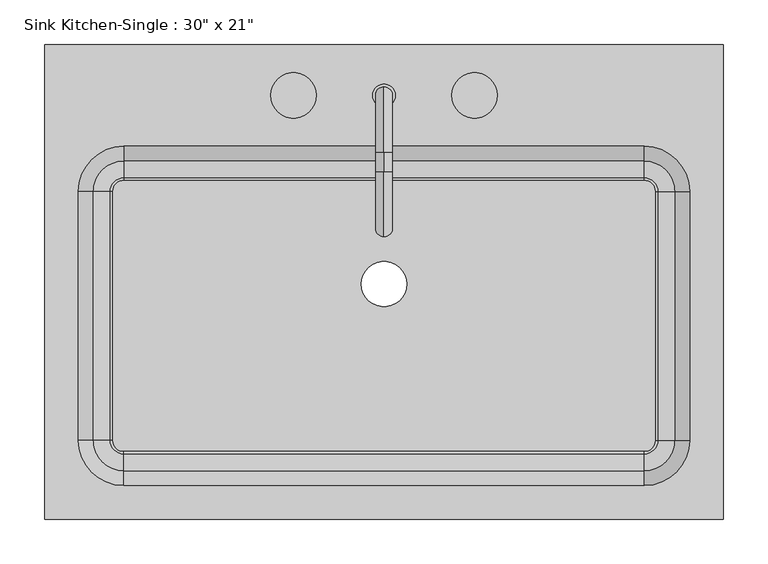
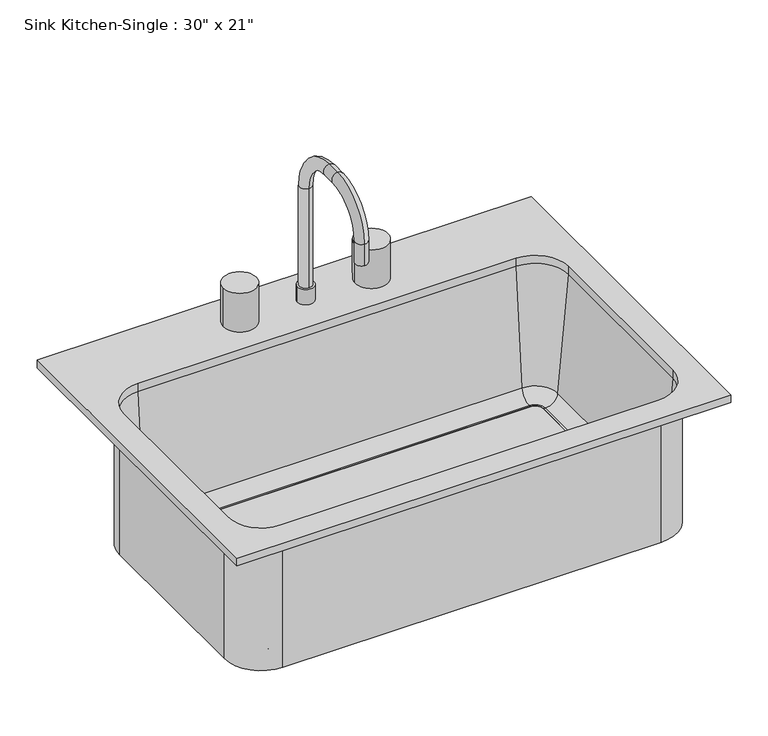
"""IFC4 building model written with IfcOpenShell, lengths in millimetres: flow terminal geometry."""

from ifc_helpers import new_model, si_unit, point, frame, frame_2d, origin, place, context, project, spatial, polyline, circle_curve, ellipse_curve, trimmed, segment, composite_curve, outline, extrude, source, transform, mapped, element, save
from ifc_brep_helpers import plane_surface, cylinder_surface, revolved_surface, advanced_brep


def flow_terminal_38af2918(model_context):
    return source(origin(), model_context, "Body", "SolidModel", [
        advanced_brep(
        [(396.6892406, 269.0454011, 927.1), (-365.3107594, 269.0454011, 927.1), (-365.3107594, -264.3545989, 927.1), (396.6892406, -264.3545989, 927.1), (307.7892406, 154.7454011, 927.1), (358.5892406, 103.9454011, 927.1), (358.5892406, -175.4545989, 927.1), (307.7892406, -226.2545989, 927.1), (-276.4107594, -226.2545989, 927.1), (-327.2107594, -175.4545989, 927.1), (-327.2107594, 103.9454011, 927.1), (-276.4107594, 154.7454011, 927.1), (396.6892406, 269.0454011, 914.4), (396.6892406, -264.3545989, 914.4), (-365.3107594, -264.3545989, 914.4), (-365.3107594, 269.0454011, 914.4), (364.9392406, 103.9454011, 914.4), (307.7892406, 161.0954011, 914.4), (-276.4107594, 161.0954011, 914.4), (-333.5607594, 103.9454011, 914.4), (-333.5607594, -175.4545989, 914.4), (-276.4107594, -232.6045989, 914.4), (307.7892406, -232.6045989, 914.4), (364.9392406, -175.4545989, 914.4), (307.7892406, 154.7454011, 914.4), (358.5892406, 103.9454011, 914.4), (358.5892406, -175.4545989, 914.4), (307.7892406, -226.2545989, 914.4), (-276.4107594, -226.2545989, 914.4), (-327.2107594, -175.4545989, 914.4), (-327.2107594, 103.9454011, 914.4), (-276.4107594, 154.7454011, 914.4), (364.9392406, 103.9454011, 698.5), (307.7892406, 161.0954011, 698.5), (320.4892406, 103.9454011, 698.5), (307.7892406, 116.6454011, 698.5), (320.4892406, 103.9454011, 708.025), (307.7892406, 116.6454011, 708.025), (323.0776588, 103.9454011, 708.025), (307.7892406, 119.2338193, 708.025), (342.0551678, 103.9454011, 725.4146831), (307.7892406, 138.2113283, 725.4146831), (364.9392406, -175.4545989, 698.5), (320.4892406, -175.4545989, 698.5), (320.4892406, -175.4545989, 708.025), (323.0776588, -175.4545989, 708.025), (342.0551678, -175.4545989, 725.4146831), (307.7892406, -232.6045989, 698.5), (307.7892406, -188.1545989, 698.5), (307.7892406, -188.1545989, 708.025), (307.7892406, -190.7430171, 708.025), (307.7892406, -209.7205261, 725.4146831), (-276.4107594, -232.6045989, 698.5), (-276.4107594, -188.1545989, 698.5), (-276.4107594, -188.1545989, 708.025), (-276.4107594, -190.7430171, 708.025), (-276.4107594, -209.7205261, 725.4146831), (-333.5607594, -175.4545989, 698.5), (-289.1107594, -175.4545989, 698.5), (-289.1107594, -175.4545989, 708.025), (-291.6991776, -175.4545989, 708.025), (-310.6766866, -175.4545989, 725.4146831), (-333.5607594, 103.9454011, 698.5), (-289.1107594, 103.9454011, 698.5), (-289.1107594, 103.9454011, 708.025), (-291.6991776, 103.9454011, 708.025), (-310.6766866, 103.9454011, 725.4146831), (-276.4107594, 161.0954011, 698.5), (-276.4107594, 116.6454011, 698.5), (-276.4107594, 116.6454011, 708.025), (-276.4107594, 119.2338193, 708.025), (-276.4107594, 138.2113283, 725.4146831)],
        [
            (0, 1),
            (1, 2),
            (2, 3),
            (3, 0),
            (4, 5, circle_curve(frame((307.7892406, 103.9454011, 927.1), z_axis=(0.0, 0.0, -1.0), x_axis=(1.0, 0.0, 0.0)), 50.8)),
            (5, 6),
            (6, 7, circle_curve(frame((307.7892406, -175.4545989, 927.1), z_axis=(0.0, 0.0, -1.0), x_axis=(1.0, 0.0, 0.0)), 50.8)),
            (7, 8),
            (8, 9, circle_curve(frame((-276.4107594, -175.4545989, 927.1), z_axis=(0.0, 0.0, -1.0), x_axis=(1.0, 0.0, 0.0)), 50.8)),
            (9, 10),
            (10, 11, circle_curve(frame((-276.4107594, 103.9454011, 927.1), z_axis=(0.0, 0.0, -1.0), x_axis=(1.0, 0.0, 0.0)), 50.8)),
            (11, 4),
            (12, 13),
            (13, 14),
            (14, 15),
            (15, 12),
            (16, 17, circle_curve(frame((307.7892406, 103.9454011, 914.4), z_axis=(0.0, 0.0, 1.0), x_axis=(0.0, 1.0, 0.0)), 57.15)),
            (17, 18),
            (18, 19, circle_curve(frame((-276.4107594, 103.9454011, 914.4), z_axis=(0.0, 0.0, 1.0), x_axis=(-1.0, 0.0, 0.0)), 57.15)),
            (19, 20),
            (20, 21, circle_curve(frame((-276.4107594, -175.4545989, 914.4), z_axis=(0.0, 0.0, 1.0), x_axis=(0.0, -1.0, 0.0)), 57.15)),
            (21, 22),
            (22, 23, circle_curve(frame((307.7892406, -175.4545989, 914.4), z_axis=(0.0, 0.0, 1.0), x_axis=(1.0, 0.0, 0.0)), 57.15)),
            (23, 16),
            (0, 12),
            (15, 1),
            (14, 2),
            (13, 3),
            (4, 24),
            (24, 25, circle_curve(frame((307.7892406, 103.9454011, 914.4), z_axis=(0.0, 0.0, -1.0), x_axis=(1.0, 0.0, 0.0)), 50.8)),
            (25, 5),
            (25, 26),
            (26, 6),
            (26, 27, circle_curve(frame((307.7892406, -175.4545989, 914.4), z_axis=(0.0, 0.0, -1.0), x_axis=(1.0, 0.0, 0.0)), 50.8)),
            (27, 7),
            (27, 28),
            (28, 8),
            (28, 29, circle_curve(frame((-276.4107594, -175.4545989, 914.4), z_axis=(0.0, 0.0, -1.0), x_axis=(1.0, 0.0, 0.0)), 50.8)),
            (29, 9),
            (29, 30),
            (30, 10),
            (30, 31, circle_curve(frame((-276.4107594, 103.9454011, 914.4), z_axis=(0.0, 0.0, -1.0), x_axis=(1.0, 0.0, 0.0)), 50.8)),
            (31, 11),
            (31, 24),
            (32, 33, circle_curve(frame((307.7892406, 103.9454011, 698.5), z_axis=(0.0, 0.0, 1.0), x_axis=(0.0, 1.0, 0.0)), 57.15)),
            (33, 17),
            (16, 32),
            (32, 34),
            (34, 35, circle_curve(frame((307.7892406, 103.9454011, 698.5), z_axis=(0.0, 0.0, 1.0), x_axis=(0.0, 1.0, 0.0)), 12.7)),
            (35, 33),
            (34, 36),
            (36, 37, circle_curve(frame((307.7892406, 103.9454011, 708.025), z_axis=(0.0, 0.0, 1.0), x_axis=(0.0, 1.0, 0.0)), 12.7)),
            (37, 35),
            (36, 38),
            (38, 39, circle_curve(frame((307.7892406, 103.9454011, 708.025), z_axis=(0.0, 0.0, 1.0), x_axis=(0.0, 1.0, 0.0)), 15.2884182)),
            (39, 37),
            (38, 40, circle_curve(frame((323.0776588, 103.9454011, 727.075), z_axis=(0.0, -1.0, 0.0), x_axis=(1.0, 0.0, 0.0)), 19.05)),
            (40, 41, circle_curve(frame((307.7892406, 103.9454011, 725.4146831), z_axis=(0.0, 0.0, 1.0), x_axis=(0.0, 1.0, 0.0)), 34.2659272)),
            (41, 39, circle_curve(frame((307.7892406, 119.2338193, 727.075), z_axis=(-1.0, 0.0, 0.0), x_axis=(0.0, 1.0, 0.0)), 19.05)),
            (40, 25),
            (24, 41),
            (23, 42),
            (42, 32),
            (42, 43),
            (43, 34),
            (43, 44),
            (44, 36),
            (44, 45),
            (45, 38),
            (45, 46, circle_curve(frame((323.0776588, -175.4545989, 727.075), z_axis=(0.0, -1.0, 0.0), x_axis=(1.0, 0.0, 0.0)), 19.05)),
            (46, 40),
            (46, 26),
            (22, 47),
            (47, 42, circle_curve(frame((307.7892406, -175.4545989, 698.5), z_axis=(0.0, 0.0, 1.0), x_axis=(1.0, 0.0, 0.0)), 57.15)),
            (47, 48),
            (48, 43, circle_curve(frame((307.7892406, -175.4545989, 698.5), z_axis=(0.0, 0.0, 1.0), x_axis=(1.0, 0.0, 0.0)), 12.7)),
            (48, 49),
            (49, 44, circle_curve(frame((307.7892406, -175.4545989, 708.025), z_axis=(0.0, 0.0, 1.0), x_axis=(1.0, 0.0, 0.0)), 12.7)),
            (49, 50),
            (50, 45, circle_curve(frame((307.7892406, -175.4545989, 708.025), z_axis=(0.0, 0.0, 1.0), x_axis=(1.0, 0.0, 0.0)), 15.2884182)),
            (50, 51, circle_curve(frame((307.7892406, -190.7430171, 727.075), z_axis=(-1.0, 0.0, 0.0), x_axis=(0.0, -1.0, 0.0)), 19.05)),
            (51, 46, circle_curve(frame((307.7892406, -175.4545989, 725.4146831), z_axis=(0.0, 0.0, 1.0), x_axis=(1.0, 0.0, 0.0)), 34.2659272)),
            (51, 27),
            (21, 52),
            (52, 47),
            (52, 53),
            (53, 48),
            (53, 54),
            (54, 49),
            (54, 55),
            (55, 50),
            (55, 56, circle_curve(frame((-276.4107594, -190.7430171, 727.075), z_axis=(-1.0, 0.0, 0.0), x_axis=(0.0, -1.0, 0.0)), 19.05)),
            (56, 51),
            (56, 28),
            (20, 57),
            (57, 52, circle_curve(frame((-276.4107594, -175.4545989, 698.5), z_axis=(0.0, 0.0, 1.0), x_axis=(0.0, -1.0, 0.0)), 57.15)),
            (57, 58),
            (58, 53, circle_curve(frame((-276.4107594, -175.4545989, 698.5), z_axis=(0.0, 0.0, 1.0), x_axis=(0.0, -1.0, 0.0)), 12.7)),
            (58, 59),
            (59, 54, circle_curve(frame((-276.4107594, -175.4545989, 708.025), z_axis=(0.0, 0.0, 1.0), x_axis=(0.0, -1.0, 0.0)), 12.7)),
            (59, 60),
            (60, 55, circle_curve(frame((-276.4107594, -175.4545989, 708.025), z_axis=(0.0, 0.0, 1.0), x_axis=(0.0, -1.0, 0.0)), 15.2884182)),
            (60, 61, circle_curve(frame((-291.6991776, -175.4545989, 727.075), z_axis=(0.0, 1.0, 0.0), x_axis=(-1.0, 0.0, 0.0)), 19.05)),
            (61, 56, circle_curve(frame((-276.4107594, -175.4545989, 725.4146831), z_axis=(0.0, 0.0, 1.0), x_axis=(0.0, -1.0, 0.0)), 34.2659272)),
            (61, 29),
            (19, 62),
            (62, 57),
            (62, 63),
            (63, 58),
            (63, 64),
            (64, 59),
            (64, 65),
            (65, 60),
            (65, 66, circle_curve(frame((-291.6991776, 103.9454011, 727.075), z_axis=(0.0, 1.0, 0.0), x_axis=(-1.0, 0.0, 0.0)), 19.05)),
            (66, 61),
            (66, 30),
            (18, 67),
            (67, 62, circle_curve(frame((-276.4107594, 103.9454011, 698.5), z_axis=(0.0, 0.0, 1.0), x_axis=(-1.0, 0.0, 0.0)), 57.15)),
            (67, 68),
            (68, 63, circle_curve(frame((-276.4107594, 103.9454011, 698.5), z_axis=(0.0, 0.0, 1.0), x_axis=(-1.0, 0.0, 0.0)), 12.7)),
            (68, 69),
            (69, 64, circle_curve(frame((-276.4107594, 103.9454011, 708.025), z_axis=(0.0, 0.0, 1.0), x_axis=(-1.0, 0.0, 0.0)), 12.7)),
            (69, 70),
            (70, 65, circle_curve(frame((-276.4107594, 103.9454011, 708.025), z_axis=(0.0, 0.0, 1.0), x_axis=(-1.0, 0.0, 0.0)), 15.2884182)),
            (70, 71, circle_curve(frame((-276.4107594, 119.2338193, 727.075), z_axis=(1.0, 0.0, 0.0), x_axis=(0.0, 1.0, 0.0)), 19.05)),
            (71, 66, circle_curve(frame((-276.4107594, 103.9454011, 725.4146831), z_axis=(0.0, 0.0, 1.0), x_axis=(-1.0, 0.0, 0.0)), 34.2659272)),
            (71, 31),
            (33, 67),
            (35, 68),
            (37, 69),
            (39, 70),
            (41, 71),
        ],
        [
            plane_surface(frame((-365.3107594, 269.0454011, 927.1), z_axis=(0.0, 0.0, 1.0), x_axis=(-1.0, 0.0, 0.0))),
            plane_surface(frame((-365.3107594, 269.0454011, 914.4), z_axis=(0.0, 0.0, -1.0), x_axis=(1.0, 0.0, 0.0))),
            plane_surface(frame((396.6892406, 269.0454011, 927.1), z_axis=(0.0, 1.0, 0.0), x_axis=(0.0, 0.0, -1.0))),
            plane_surface(frame((-365.3107594, 269.0454011, 927.1), z_axis=(-1.0, 0.0, 0.0), x_axis=(0.0, 0.0, -1.0))),
            plane_surface(frame((-365.3107594, -264.3545989, 927.1), z_axis=(0.0, -1.0, 0.0), x_axis=(0.0, 0.0, -1.0))),
            plane_surface(frame((396.6892406, -264.3545989, 927.1), z_axis=(1.0, 0.0, 0.0), x_axis=(0.0, 0.0, -1.0))),
            revolved_surface(polyline([(358.58924060000004, 103.9454011, 914.4), (358.58924060000004, 103.9454011, 927.1)]), (307.7892406, 103.9454011, 0.0), (0.0, 0.0, -1.0)),
            plane_surface(frame((358.5892406, 103.9454011, 927.1), z_axis=(-1.0, 0.0, 0.0), x_axis=(0.0, 0.0, -1.0))),
            revolved_surface(polyline([(358.58924060000004, -175.4545989, 914.4), (358.58924060000004, -175.4545989, 927.1)]), (307.7892406, -175.4545989, 0.0), (0.0, 0.0, -1.0)),
            plane_surface(frame((307.7892406, -226.2545989, 927.1), z_axis=(0.0, 1.0, 0.0), x_axis=(0.0, 0.0, -1.0))),
            revolved_surface(polyline([(-225.6107594, -175.4545989, 914.4), (-225.6107594, -175.4545989, 927.1)]), (-276.4107594, -175.4545989, 0.0), (0.0, 0.0, -1.0)),
            plane_surface(frame((-327.2107594, -175.4545989, 927.1), z_axis=(1.0, 0.0, 0.0), x_axis=(0.0, 0.0, -1.0))),
            revolved_surface(polyline([(-225.6107594, 103.9454011, 914.4), (-225.6107594, 103.9454011, 927.1)]), (-276.4107594, 103.9454011, 0.0), (0.0, 0.0, -1.0)),
            plane_surface(frame((-276.4107594, 154.7454011, 927.1), z_axis=(0.0, -1.0, 0.0), x_axis=(0.0, 0.0, -1.0))),
            cylinder_surface(frame((307.7892406, 103.9454011, 0.0), z_axis=(0.0, 0.0, -1.0), x_axis=(0.0, 1.0, 0.0)), 57.15),
            plane_surface(frame((307.7892406, 103.9454011, 698.5), z_axis=(0.0, 0.0, -1.0), x_axis=(0.0, 1.0, 0.0))),
            revolved_surface(polyline([(307.7892406, 116.6454011, 698.5), (307.7892406, 116.6454011, 708.025)]), (307.7892406, 103.9454011, 0.0), (0.0, 0.0, -1.0)),
            plane_surface(frame((307.7892406, 103.9454011, 708.025), z_axis=(0.0, 0.0, 1.0), x_axis=(0.0, 1.0, 0.0))),
            revolved_surface(trimmed(ellipse_curve(frame((307.7892406, 119.2338193, 727.075), z_axis=(1.0, 0.0, 0.0), x_axis=(0.0, 1.0, 0.0)), 19.05, 19.05), [point((307.7892406, 119.2338193, 708.025))], [point((307.7892406, 138.2113283, 725.4146831))], True, "CARTESIAN"), (307.7892406, 103.9454011, 0.0), (0.0, 0.0, -1.0)),
            revolved_surface(polyline([(307.7892406, 138.2113283, 725.4146831), (307.7892406, 154.7454011, 914.4)]), (307.7892406, 103.9454011, 0.0), (0.0, 0.0, -1.0)),
            plane_surface(frame((364.9392406, 103.9454011, 914.4), z_axis=(1.0, 0.0, 0.0), x_axis=(0.0, -1.0, 0.0))),
            plane_surface(frame((364.9392406, 103.9454011, 698.5), z_axis=(0.0, 0.0, -1.0), x_axis=(0.0, -1.0, 0.0))),
            plane_surface(frame((320.4892406, 103.9454011, 698.5), z_axis=(-1.0, 0.0, 0.0), x_axis=(0.0, -1.0, 0.0))),
            plane_surface(frame((320.4892406, 103.9454011, 708.025), z_axis=(0.0, 0.0, 1.0), x_axis=(0.0, -1.0, 0.0))),
            revolved_surface(polyline([(342.1276588, -175.45459889999998, 727.075), (342.1276588, 103.9454011, 727.075)]), (323.0776588, 103.9454011, 727.075), (0.0, -1.0, 0.0)),
            plane_surface(frame((342.0551678, 103.9454011, 725.4146831), z_axis=(-0.9961946980917442, 0.0, 0.08715574274767306), x_axis=(0.0, -1.0, 0.0))),
            cylinder_surface(frame((307.7892406, -175.4545989, 0.0), z_axis=(0.0, 0.0, -1.0), x_axis=(1.0, 0.0, 0.0)), 57.15),
            plane_surface(frame((307.7892406, -175.4545989, 698.5), z_axis=(0.0, 0.0, -1.0), x_axis=(1.0, 0.0, 0.0))),
            revolved_surface(polyline([(320.4892406, -175.4545989, 698.5), (320.4892406, -175.4545989, 708.025)]), (307.7892406, -175.4545989, 0.0), (0.0, 0.0, -1.0)),
            plane_surface(frame((307.7892406, -175.4545989, 708.025), z_axis=(0.0, 0.0, 1.0), x_axis=(1.0, 0.0, 0.0))),
            revolved_surface(trimmed(ellipse_curve(frame((323.0776588, -175.4545989, 727.075), z_axis=(0.0, -1.0, 0.0), x_axis=(1.0, 0.0, 0.0)), 19.05, 19.05), [point((323.0776588, -175.4545989, 708.025))], [point((342.0551678, -175.4545989, 725.4146831))], True, "CARTESIAN"), (307.7892406, -175.4545989, 0.0), (0.0, 0.0, -1.0)),
            revolved_surface(polyline([(342.0551678, -175.4545989, 725.4146831), (358.5892406, -175.4545989, 914.4)]), (307.7892406, -175.4545989, 0.0), (0.0, 0.0, -1.0)),
            plane_surface(frame((307.7892406, -232.6045989, 914.4), z_axis=(0.0, -1.0, 0.0), x_axis=(-1.0, 0.0, 0.0))),
            plane_surface(frame((307.7892406, -232.6045989, 698.5), z_axis=(0.0, 0.0, -1.0), x_axis=(-1.0, 0.0, 0.0))),
            plane_surface(frame((307.7892406, -188.1545989, 698.5), z_axis=(0.0, 1.0, 0.0), x_axis=(-1.0, 0.0, 0.0))),
            plane_surface(frame((307.7892406, -188.1545989, 708.025), z_axis=(0.0, 0.0, 1.0), x_axis=(-1.0, 0.0, 0.0))),
            revolved_surface(polyline([(-276.4107594, -209.79301710000001, 727.075), (307.7892406, -209.79301710000001, 727.075)]), (307.7892406, -190.7430171, 727.075), (-1.0, 0.0, 0.0)),
            plane_surface(frame((307.7892406, -209.7205261, 725.4146831), z_axis=(0.0, 0.9961946980917442, 0.08715574274767306), x_axis=(-1.0, 0.0, 0.0))),
            cylinder_surface(frame((-276.4107594, -175.4545989, 0.0), z_axis=(0.0, 0.0, -1.0), x_axis=(0.0, -1.0, 0.0)), 57.15),
            plane_surface(frame((-276.4107594, -175.4545989, 698.5), z_axis=(0.0, 0.0, -1.0), x_axis=(0.0, -1.0, 0.0))),
            revolved_surface(polyline([(-276.4107594, -188.1545989, 698.5), (-276.4107594, -188.1545989, 708.025)]), (-276.4107594, -175.4545989, 0.0), (0.0, 0.0, -1.0)),
            plane_surface(frame((-276.4107594, -175.4545989, 708.025), z_axis=(0.0, 0.0, 1.0), x_axis=(0.0, -1.0, 0.0))),
            revolved_surface(trimmed(ellipse_curve(frame((-276.4107594, -190.7430171, 727.075), z_axis=(-1.0, 0.0, 0.0), x_axis=(0.0, -1.0, 0.0)), 19.05, 19.05), [point((-276.4107594, -190.7430171, 708.025))], [point((-276.4107594, -209.7205261, 725.4146831))], True, "CARTESIAN"), (-276.4107594, -175.4545989, 0.0), (0.0, 0.0, -1.0)),
            revolved_surface(polyline([(-276.4107594, -209.7205261, 725.4146831), (-276.4107594, -226.2545989, 914.4)]), (-276.4107594, -175.4545989, 0.0), (0.0, 0.0, -1.0)),
            plane_surface(frame((-333.5607594, -175.4545989, 914.4), z_axis=(-1.0, 0.0, 0.0), x_axis=(0.0, 1.0, 0.0))),
            plane_surface(frame((-333.5607594, -175.4545989, 698.5), z_axis=(0.0, 0.0, -1.0), x_axis=(0.0, 1.0, 0.0))),
            plane_surface(frame((-289.1107594, -175.4545989, 698.5), z_axis=(1.0, 0.0, 0.0), x_axis=(0.0, 1.0, 0.0))),
            plane_surface(frame((-289.1107594, -175.4545989, 708.025), z_axis=(0.0, 0.0, 1.0), x_axis=(0.0, 1.0, 0.0))),
            revolved_surface(polyline([(-310.7491776, 103.94540109999997, 727.075), (-310.7491776, -175.4545989, 727.075)]), (-291.6991776, -175.4545989, 727.075), (0.0, 1.0, 0.0)),
            plane_surface(frame((-310.6766866, -175.4545989, 725.4146831), z_axis=(0.9961946980917442, 0.0, 0.08715574274767306), x_axis=(0.0, 1.0, 0.0))),
            cylinder_surface(frame((-276.4107594, 103.9454011, 0.0), z_axis=(0.0, 0.0, -1.0), x_axis=(-1.0, 0.0, 0.0)), 57.15),
            plane_surface(frame((-276.4107594, 103.9454011, 698.5), z_axis=(0.0, 0.0, -1.0), x_axis=(-1.0, 0.0, 0.0))),
            revolved_surface(polyline([(-289.1107594, 103.9454011, 698.5), (-289.1107594, 103.9454011, 708.025)]), (-276.4107594, 103.9454011, 0.0), (0.0, 0.0, -1.0)),
            plane_surface(frame((-276.4107594, 103.9454011, 708.025), z_axis=(0.0, 0.0, 1.0), x_axis=(-1.0, 0.0, 0.0))),
            revolved_surface(trimmed(ellipse_curve(frame((-291.6991776, 103.9454011, 727.075), z_axis=(0.0, 1.0, 0.0), x_axis=(-1.0, 0.0, 0.0)), 19.05, 19.05), [point((-291.6991776, 103.9454011, 708.025))], [point((-310.6766866, 103.9454011, 725.4146831))], True, "CARTESIAN"), (-276.4107594, 103.9454011, 0.0), (0.0, 0.0, -1.0)),
            revolved_surface(polyline([(-310.6766866, 103.9454011, 725.4146831), (-327.2107594, 103.9454011, 914.4)]), (-276.4107594, 103.9454011, 0.0), (0.0, 0.0, -1.0)),
            plane_surface(frame((-276.4107594, 161.0954011, 914.4), z_axis=(0.0, 1.0, 0.0), x_axis=(1.0, 0.0, 0.0))),
            plane_surface(frame((-276.4107594, 161.0954011, 698.5), z_axis=(0.0, 0.0, -1.0), x_axis=(1.0, 0.0, 0.0))),
            plane_surface(frame((-276.4107594, 116.6454011, 698.5), z_axis=(0.0, -1.0, 0.0), x_axis=(1.0, 0.0, 0.0))),
            plane_surface(frame((-276.4107594, 116.6454011, 708.025), z_axis=(0.0, 0.0, 1.0), x_axis=(1.0, 0.0, 0.0))),
            revolved_surface(polyline([(307.7892406, 138.2838193, 727.075), (-276.4107594, 138.2838193, 727.075)]), (-276.4107594, 119.2338193, 727.075), (1.0, 0.0, 0.0)),
            plane_surface(frame((-276.4107594, 138.2113283, 725.4146831), z_axis=(0.0, -0.9961946980917442, 0.08715574274767306), x_axis=(1.0, 0.0, 0.0))),
        ],
        [
            (0, [[1, 2, 3, 4], [5, 6, 7, 8, 9, 10, 11, 12]]),
            (1, [[13, 14, 15, 16], [17, 18, 19, 20, 21, 22, 23, 24]]),
            (2, [[-1, 25, -16, 26]]),
            (3, [[-2, -26, -15, 27]]),
            (4, [[-3, -27, -14, 28]]),
            (5, [[-4, -28, -13, -25]]),
            (6, [[-5, 29, 30, 31]]),
            (7, [[-6, -31, 32, 33]]),
            (8, [[-7, -33, 34, 35]]),
            (9, [[-8, -35, 36, 37]]),
            (10, [[-9, -37, 38, 39]]),
            (11, [[-10, -39, 40, 41]]),
            (12, [[-11, -41, 42, 43]]),
            (13, [[-12, -43, 44, -29]]),
            (14, [[45, 46, -17, 47]]),
            (15, [[-45, 48, 49, 50]]),
            (16, [[-49, 51, 52, 53]]),
            (17, [[-52, 54, 55, 56]]),
            (18, [[-55, 57, 58, 59]]),
            (19, [[-58, 60, -30, 61]]),
            (20, [[-47, -24, 62, 63]]),
            (21, [[-48, -63, 64, 65]]),
            (22, [[-51, -65, 66, 67]]),
            (23, [[-54, -67, 68, 69]]),
            (24, [[-57, -69, 70, 71]]),
            (25, [[-60, -71, 72, -32]]),
            (26, [[-62, -23, 73, 74]]),
            (27, [[-64, -74, 75, 76]]),
            (28, [[-66, -76, 77, 78]]),
            (29, [[-68, -78, 79, 80]]),
            (30, [[-70, -80, 81, 82]]),
            (31, [[-72, -82, 83, -34]]),
            (32, [[-73, -22, 84, 85]]),
            (33, [[-75, -85, 86, 87]]),
            (34, [[-77, -87, 88, 89]]),
            (35, [[-79, -89, 90, 91]]),
            (36, [[-81, -91, 92, 93]]),
            (37, [[-83, -93, 94, -36]]),
            (38, [[-84, -21, 95, 96]]),
            (39, [[-86, -96, 97, 98]]),
            (40, [[-88, -98, 99, 100]]),
            (41, [[-90, -100, 101, 102]]),
            (42, [[-92, -102, 103, 104]]),
            (43, [[-94, -104, 105, -38]]),
            (44, [[-95, -20, 106, 107]]),
            (45, [[-97, -107, 108, 109]]),
            (46, [[-99, -109, 110, 111]]),
            (47, [[-101, -111, 112, 113]]),
            (48, [[-103, -113, 114, 115]]),
            (49, [[-105, -115, 116, -40]]),
            (50, [[-106, -19, 117, 118]]),
            (51, [[-108, -118, 119, 120]]),
            (52, [[-110, -120, 121, 122]]),
            (53, [[-112, -122, 123, 124]]),
            (54, [[-114, -124, 125, 126]]),
            (55, [[-116, -126, 127, -42]]),
            (56, [[-46, 128, -117, -18]]),
            (57, [[-50, 129, -119, -128]]),
            (58, [[-53, 130, -121, -129]]),
            (59, [[-56, 131, -123, -130]]),
            (60, [[-59, 132, -125, -131]]),
            (61, [[-61, -44, -127, -132]]),
        ],
    ),
        advanced_brep(
        [(2.9892406, 211.8954011, 927.1), (28.3892406, 211.8954011, 927.1), (15.6892406, 221.4204011, 1114.425), (15.6892406, 202.3704011, 1114.425), (15.6892406, 202.3704011, 952.5), (15.6892406, 221.4204011, 952.5), (15.6892406, 148.3954011, 1187.45), (15.6892406, 148.3954011, 1168.4), (15.6892406, 126.1704011, 1187.45), (15.6892406, 126.1704011, 1168.4), (15.6892406, 53.1454011, 1114.425), (15.6892406, 72.1954011, 1114.425), (15.6892406, 53.1454011, 1079.5), (15.6892406, 72.1954011, 1079.5), (2.9892406, 211.8954011, 952.5), (28.3892406, 211.8954011, 952.5)],
        [
            (0, 1, circle_curve(frame((15.6892406, 211.8954011, 927.1), z_axis=(0.0, 0.0, -1.0), x_axis=(1.0, 0.0, 0.0)), 12.7)),
            (1, 0, circle_curve(frame((15.6892406, 211.8954011, 927.1), z_axis=(0.0, 0.0, -1.0), x_axis=(1.0, 0.0, 0.0)), 12.7)),
            (2, 3, circle_curve(frame((15.6892406, 211.8954011, 1114.425), z_axis=(0.0, 0.0, -1.0), x_axis=(0.0, -1.0, 0.0)), 9.525)),
            (3, 4),
            (4, 5, circle_curve(frame((15.6892406, 211.8954011, 952.5), z_axis=(0.0, 0.0, 1.0), x_axis=(0.0, -1.0, 0.0)), 9.525)),
            (5, 2),
            (3, 2, circle_curve(frame((15.6892406, 211.8954011, 1114.425), z_axis=(0.0, 0.0, -1.0), x_axis=(0.0, -1.0, 0.0)), 9.525)),
            (5, 4, circle_curve(frame((15.6892406, 211.8954011, 952.5), z_axis=(0.0, 0.0, 1.0), x_axis=(0.0, -1.0, 0.0)), 9.525)),
            (2, 6, circle_curve(frame((15.6892406, 148.3954011, 1114.425), z_axis=(1.0, 0.0, 0.0), x_axis=(0.0, 1.0, 0.0)), 73.025)),
            (6, 7, circle_curve(frame((15.6892406, 148.3954011, 1177.925), z_axis=(0.0, 1.0, 0.0), x_axis=(0.0, 0.0, -1.0)), 9.525)),
            (7, 3, circle_curve(frame((15.6892406, 148.3954011, 1114.425), z_axis=(-1.0, 0.0, 0.0), x_axis=(0.0, 1.0, 0.0)), 53.975)),
            (7, 6, circle_curve(frame((15.6892406, 148.3954011, 1177.925), z_axis=(0.0, 1.0, 0.0), x_axis=(0.0, 0.0, -1.0)), 9.525)),
            (6, 8),
            (8, 9, circle_curve(frame((15.6892406, 126.1704011, 1177.925), z_axis=(0.0, 1.0, 0.0), x_axis=(0.0, 0.0, -1.0)), 9.525)),
            (9, 7),
            (9, 8, circle_curve(frame((15.6892406, 126.1704011, 1177.925), z_axis=(0.0, 1.0, 0.0), x_axis=(0.0, 0.0, -1.0)), 9.525)),
            (8, 10, circle_curve(frame((15.6892406, 126.1704011, 1114.425), z_axis=(1.0, 0.0, 0.0), x_axis=(0.0, 0.0, 1.0)), 73.025)),
            (10, 11, circle_curve(frame((15.6892406, 62.6704011, 1114.425), z_axis=(0.0, 0.0, 1.0), x_axis=(0.0, 1.0, 0.0)), 9.525)),
            (11, 9, circle_curve(frame((15.6892406, 126.1704011, 1114.425), z_axis=(-1.0, 0.0, 0.0), x_axis=(0.0, 0.0, 1.0)), 53.975)),
            (11, 10, circle_curve(frame((15.6892406, 62.6704011, 1114.425), z_axis=(0.0, 0.0, 1.0), x_axis=(0.0, 1.0, 0.0)), 9.525)),
            (12, 13, circle_curve(frame((15.6892406, 62.6704011, 1079.5), z_axis=(0.0, 0.0, -1.0), x_axis=(0.0, 1.0, 0.0)), 9.525)),
            (13, 12, circle_curve(frame((15.6892406, 62.6704011, 1079.5), z_axis=(0.0, 0.0, -1.0), x_axis=(0.0, 1.0, 0.0)), 9.525)),
            (10, 12),
            (13, 11),
            (14, 15, circle_curve(frame((15.6892406, 211.8954011, 952.5), z_axis=(0.0, 0.0, 1.0), x_axis=(1.0, 0.0, 0.0)), 12.7)),
            (15, 14, circle_curve(frame((15.6892406, 211.8954011, 952.5), z_axis=(0.0, 0.0, 1.0), x_axis=(1.0, 0.0, 0.0)), 12.7)),
            (14, 0),
            (1, 15),
        ],
        [
            plane_surface(frame((15.6892406, 202.3704011, 927.1), z_axis=(0.0, 0.0, -1.0), x_axis=(1.0, 0.0, 0.0))),
            cylinder_surface(frame((15.6892406, 211.8954011, 927.1), z_axis=(0.0, 0.0, -1.0), x_axis=(0.0, -1.0, 0.0)), 9.525),
            revolved_surface(trimmed(ellipse_curve(frame((15.6892406, 211.8954011, 1114.425), z_axis=(0.0, 0.0, -1.0), x_axis=(0.0, -1.0, 0.0)), 9.525, 9.525), [point((15.6892406, 221.4204011, 1114.425))], [point((15.6892406, 202.3704011, 1114.425))], True, "CARTESIAN"), (15.6892406, 148.3954011, 1114.425), (1.0, 0.0, 0.0)),
            revolved_surface(trimmed(ellipse_curve(frame((15.6892406, 211.8954011, 1114.425), z_axis=(0.0, 0.0, -1.0), x_axis=(0.0, -1.0, 0.0)), 9.525, 9.525), [point((15.6892406, 202.3704011, 1114.425))], [point((15.6892406, 221.4204011, 1114.425))], True, "CARTESIAN"), (15.6892406, 148.3954011, 1114.425), (1.0, 0.0, 0.0)),
            cylinder_surface(frame((15.6892406, 148.3954011, 1177.925), z_axis=(0.0, 1.0, 0.0), x_axis=(0.0, 0.0, -1.0)), 9.525),
            revolved_surface(trimmed(ellipse_curve(frame((15.6892406, 126.1704011, 1177.925), z_axis=(0.0, 1.0, 0.0), x_axis=(0.0, 0.0, -1.0)), 9.525, 9.525), [point((15.6892406, 126.1704011, 1187.45))], [point((15.6892406, 126.1704011, 1168.4))], True, "CARTESIAN"), (15.6892406, 126.1704011, 1114.425), (1.0, 0.0, 0.0)),
            revolved_surface(trimmed(ellipse_curve(frame((15.6892406, 126.1704011, 1177.925), z_axis=(0.0, 1.0, 0.0), x_axis=(0.0, 0.0, -1.0)), 9.525, 9.525), [point((15.6892406, 126.1704011, 1168.4))], [point((15.6892406, 126.1704011, 1187.45))], True, "CARTESIAN"), (15.6892406, 126.1704011, 1114.425), (1.0, 0.0, 0.0)),
            plane_surface(frame((15.6892406, 53.1454011, 1079.5), z_axis=(0.0, 0.0, -1.0), x_axis=(-1.0, 0.0, 0.0))),
            cylinder_surface(frame((15.6892406, 62.6704011, 1114.425), z_axis=(0.0, 0.0, 1.0), x_axis=(0.0, 1.0, 0.0)), 9.525),
            plane_surface(frame((28.3892406, 211.8954011, 952.5), z_axis=(0.0, 0.0, 1.0), x_axis=(0.0, 1.0, 0.0))),
            cylinder_surface(frame((15.6892406, 211.8954011, 927.1), z_axis=(0.0, 0.0, 1.0), x_axis=(1.0, 0.0, 0.0)), 12.7),
        ],
        [
            (0, [[1, 2]]),
            (1, [[3, 4, 5, 6]]),
            (1, [[7, -6, 8, -4]]),
            (2, [[-3, 9, 10, 11]]),
            (3, [[-7, -11, 12, -9]]),
            (4, [[-10, 13, 14, 15]]),
            (4, [[-12, -15, 16, -13]]),
            (5, [[-14, 17, 18, 19]]),
            (6, [[-16, -19, 20, -17]]),
            (7, [[21, 22]]),
            (8, [[-18, 23, -22, 24]]),
            (8, [[-20, -24, -21, -23]]),
            (9, [[25, 26], [-5, -8]]),
            (10, [[-25, 27, -2, 28]]),
            (10, [[-26, -28, -1, -27]]),
        ],
    ),
        extrude(outline(composite_curve([segment(trimmed(circle_curve(frame_2d((-85.9107594, 211.8954011)), 25.4), [point((-111.3107594, 211.8954011))], [point((-60.5107594, 211.8954011))], False, "CARTESIAN"), True, "CONTINUOUS"), segment(trimmed(circle_curve(frame_2d((-85.9107594, 211.8954011)), 25.4), [point((-60.5107594, 211.8954011))], [point((-111.3107594, 211.8954011))], False, "CARTESIAN"), True, "CONTINUOUS")], self_intersect=False)), frame((0.0, 0.0, 927.1), z_axis=(0.0, 0.0, 1.0), x_axis=(1.0, 0.0, 0.0)), (0.0, 0.0, 1.0), 63.5),
        extrude(outline(composite_curve([segment(trimmed(circle_curve(frame_2d((117.2892406, 211.8954011)), 25.4), [point((91.8892406, 211.8954011))], [point((142.6892406, 211.8954011))], False, "CARTESIAN"), True, "CONTINUOUS"), segment(trimmed(circle_curve(frame_2d((117.2892406, 211.8954011)), 25.4), [point((142.6892406, 211.8954011))], [point((91.8892406, 211.8954011))], False, "CARTESIAN"), True, "CONTINUOUS")], self_intersect=False)), frame((0.0, 0.0, 927.1), z_axis=(0.0, 0.0, 1.0), x_axis=(1.0, 0.0, 0.0)), (0.0, 0.0, 1.0), 63.5),
        extrude(outline(composite_curve([segment(trimmed(circle_curve(frame_2d((307.7892406, 103.9454011)), 12.7), [point((307.7892406, 116.6454011))], [point((320.4892406, 103.9454011))], False, "CARTESIAN"), True, "CONTINUOUS"), segment(polyline([(320.4892406, 103.9454011), (320.4892406, -175.4545989)]), True, "CONTINUOUS"), segment(trimmed(circle_curve(frame_2d((307.7892406, -175.4545989)), 12.7), [point((320.4892406, -175.4545989))], [point((307.7892406, -188.1545989))], False, "CARTESIAN"), True, "CONTINUOUS"), segment(polyline([(307.7892406, -188.1545989), (-276.4107594, -188.1545989)]), True, "CONTINUOUS"), segment(trimmed(circle_curve(frame_2d((-276.4107594, -175.4545989)), 12.7), [point((-276.4107594, -188.1545989))], [point((-289.1107594, -175.4545989))], False, "CARTESIAN"), True, "CONTINUOUS"), segment(polyline([(-289.1107594, -175.4545989), (-289.1107594, 103.9454011)]), True, "CONTINUOUS"), segment(trimmed(circle_curve(frame_2d((-276.4107594, 103.9454011)), 12.7), [point((-289.1107594, 103.9454011))], [point((-276.4107594, 116.6454011))], False, "CARTESIAN"), True, "CONTINUOUS"), segment(polyline([(-276.4107594, 116.6454011), (307.7892406, 116.6454011)]), True, "CONTINUOUS")], self_intersect=False), holes=[composite_curve([segment(trimmed(circle_curve(frame_2d((15.6892406, 0.0)), 25.4), [point((-9.7107594, 0.0))], [point((41.0892406, 0.0))], True, "CARTESIAN"), True, "CONTINUOUS"), segment(trimmed(circle_curve(frame_2d((15.6892406, 0.0)), 25.4), [point((41.0892406, 0.0))], [point((-9.7107594, 0.0))], True, "CARTESIAN"), True, "CONTINUOUS")], self_intersect=False)]), frame((0.0, 0.0, 698.5), z_axis=(0.0, 0.0, 1.0), x_axis=(1.0, 0.0, 0.0)), (0.0, 0.0, 1.0), 9.525),
    ])


if __name__ == "__main__":
    model = new_model("IFC4")
    model_context = context("Model", 3, world=origin())
    ifc_project = project(units=[si_unit("LENGTHUNIT", "METRE", prefix="MILLI")], contexts=[model_context])
    site = spatial("IfcSite", under=ifc_project)
    building = spatial("IfcBuilding", under=site)
    placement = place(None, origin())
    flow_terminal_shape = flow_terminal_38af2918(model_context)
    element("IfcFlowTerminal", 1, ObjectType="Sink Kitchen-Single : 30\" x 21\"", at=placement, inside=building, context=model_context, shape_type="MappedRepresentation", body=[
        mapped(flow_terminal_shape, transform((0.0, 0.0, 0.0), x_axis=(1.0, 0.0, 0.0), y_axis=(0.0, 1.0, 0.0), z_axis=(0.0, 0.0, 1.0))),
    ])
    save(model, "model.ifc")

# Revit data of these elements
# Type "Sink Kitchen-Single : 30\" x 21\""
#   Assembly Code = "D2010410"
#   Counter Height = 3' - 0"
#   Depth = 1' - 9"
#   Width = 2' - 6"
#   Faucet Material = none
#   Sink Material = none
